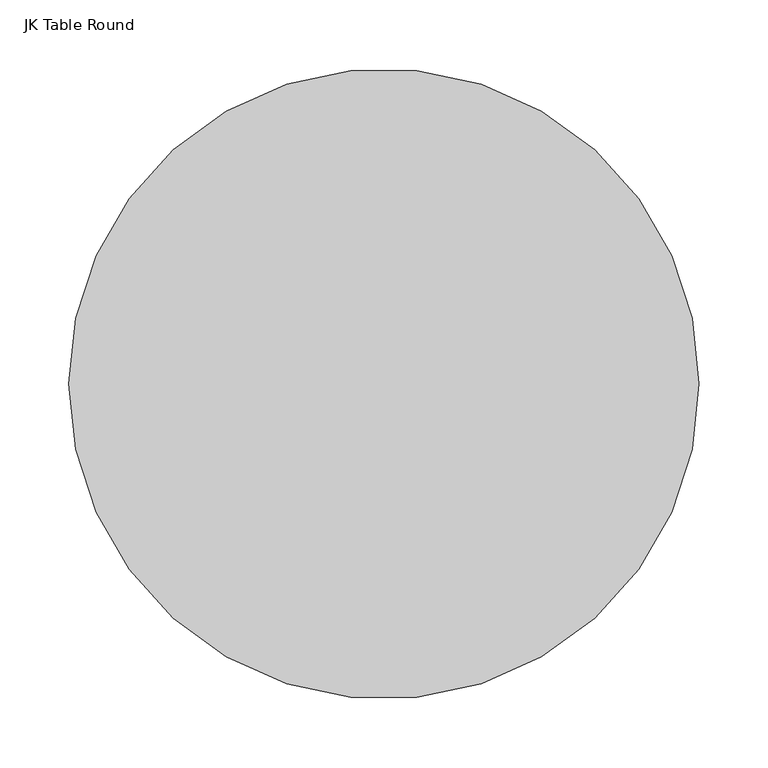
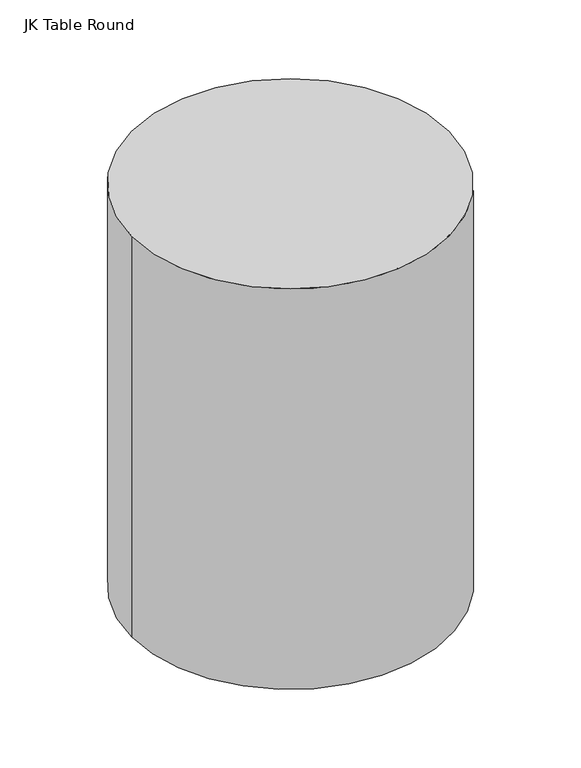
"""IFC4 building model written with IfcOpenShell, lengths in millimetres: furniture geometry, JK Table Round : Counsel End Table."""

import ifcopenshell
import ifcopenshell.guid

model = None  # the IFC model being written
_history = None  # IfcOwnerHistory: only IFC2X3 demands one
_inside = {}  # id of a spatial element -> (the spatial element, [elements in it])
_under = {}  # id of a project, library or spatial element -> (it, [spatial elements below it])
_declared = {}  # id of a project -> (the project, [libraries it declares])
_typed = {}  # id of a type object -> (the type object, [elements of that type])
_made_of = {}  # id of a material, layer set ... -> (it, [elements and type objects made of it])


def new_model(schema):
    """Start an empty IFC model of exactly this schema.

    Asked for "IFC4X3", IfcOpenShell would pick the latest addendum, in which some entities
    have other attributes; the version numbers below select the first issue.
    IFC2X3 requires an IfcOwnerHistory on every rooted entity: one is made here for all.
    """
    global model, _history
    if schema == "IFC4X3":
        model = ifcopenshell.file(schema_version=(4, 3, 0, 0))
    else:
        model = ifcopenshell.file(schema=schema)
    _inside.clear()
    _under.clear()
    _declared.clear()
    _typed.clear()
    _made_of.clear()
    _history = None
    if model.schema == "IFC2X3":
        org = make("IfcOrganization", Name="unknown")
        user = make(
            "IfcPersonAndOrganization",
            ThePerson=make("IfcPerson", FamilyName="unknown"),
            TheOrganization=org,
        )
        app = make(
            "IfcApplication",
            ApplicationDeveloper=org,
            Version="unknown",
            ApplicationFullName="unknown",
            ApplicationIdentifier="unknown",
        )
        _history = make(
            "IfcOwnerHistory",
            OwningUser=user,
            OwningApplication=app,
            ChangeAction="ADDED",
            CreationDate=0,
        )
    return model


def make(cls, **values):
    """One entity of the class cls with the attributes given. An attribute that is None is left unset."""
    return model.create_entity(
        cls, **{name: value for name, value in values.items() if value is not None}
    )


def rooted(cls, **values):
    """An entity with a GlobalId (a new one), such as an element, a storey or a relation."""
    return make(cls, GlobalId=ifcopenshell.guid.new(), OwnerHistory=_history, **values)


def si_unit(unit_type, name, prefix=None):
    """IfcSIUnit, for example si_unit("LENGTHUNIT", "METRE", prefix="MILLI")."""
    return make("IfcSIUnit", UnitType=unit_type, Prefix=prefix, Name=name)


def assignment(units):
    """IfcUnitAssignment: the units of a project."""
    return None if units is None else make("IfcUnitAssignment", Units=units)


def point(xyz):
    """IfcCartesianPoint."""
    return None if xyz is None else make("IfcCartesianPoint", Coordinates=xyz)


def direction(xyz):
    """IfcDirection."""
    return None if xyz is None else make("IfcDirection", DirectionRatios=xyz)


def frame(location, z_axis=None, x_axis=None):
    """IfcAxis2Placement3D, a coordinate frame: its origin and axes. An axis left out is left unset."""
    return make(
        "IfcAxis2Placement3D",
        Location=point(location),
        Axis=direction(z_axis),
        RefDirection=direction(x_axis),
    )


def frame_2d(location, x_axis=None):
    """IfcAxis2Placement2D, a coordinate frame in the plane: its origin and x axis."""
    return make(
        "IfcAxis2Placement2D", Location=point(location), RefDirection=direction(x_axis)
    )


def origin():
    """The frame at (0, 0, 0) with its axes left unset."""
    return frame((0.0, 0.0, 0.0))


def origin_with_axes():
    """The frame at (0, 0, 0) with the z axis (0, 0, 1) and the x axis (1, 0, 0) written out."""
    return frame((0.0, 0.0, 0.0), z_axis=(0.0, 0.0, 1.0), x_axis=(1.0, 0.0, 0.0))


def place(relative_to, where):
    """IfcLocalPlacement: puts the frame where relative to a parent placement (None: the world)."""
    return make(
        "IfcLocalPlacement", PlacementRelTo=relative_to, RelativePlacement=where
    )


def context(
    kind, dimensions, precision=None, world=None, true_north=None, identifier=None
):
    """IfcGeometricRepresentationContext, for example the 3D "Model" context."""
    return make(
        "IfcGeometricRepresentationContext",
        ContextIdentifier=identifier,
        ContextType=kind,
        CoordinateSpaceDimension=dimensions,
        Precision=precision,
        WorldCoordinateSystem=world,
        TrueNorth=true_north,
    )


def project(units=None, contexts=None):
    """IfcProject with its units and contexts."""
    return rooted(
        "IfcProject",
        Name="project",
        RepresentationContexts=contexts,
        UnitsInContext=assignment(units),
    )


def spatial(cls, under=None, at=None, **own):
    """A site, building, storey or space (cls), placed at a placement, below another one or the project."""
    s = rooted(cls, ObjectPlacement=at, **own)
    if under is not None:
        _under.setdefault(under.id(), (under, []))[1].append(s)
    return s


def circle_curve(where, radius):
    """IfcCircle in the frame where."""
    return make("IfcCircle", Position=where, Radius=radius)


def trimmed(basis, trim1, trim2, sense, master):
    """IfcTrimmedCurve: the piece of a basis curve between two trims."""
    return make(
        "IfcTrimmedCurve",
        BasisCurve=basis,
        Trim1=trim1,
        Trim2=trim2,
        SenseAgreement=sense,
        MasterRepresentation=master,
    )


def segment(curve, same_sense, transition):
    """IfcCompositeCurveSegment."""
    return make(
        "IfcCompositeCurveSegment",
        Transition=transition,
        SameSense=same_sense,
        ParentCurve=curve,
    )


def composite_curve(segments, self_intersect=None):
    """IfcCompositeCurve: segments joined end to end."""
    return make("IfcCompositeCurve", Segments=segments, SelfIntersect=self_intersect)


def outline(outer, holes=None, kind="AREA"):
    """IfcArbitraryClosedProfileDef: a profile drawn as a closed curve; with holes, ...WithVoids."""
    if holes is None:
        return make("IfcArbitraryClosedProfileDef", ProfileType=kind, OuterCurve=outer)
    return make(
        "IfcArbitraryProfileDefWithVoids",
        ProfileType=kind,
        OuterCurve=outer,
        InnerCurves=holes,
    )


def extrude(swept, where, along, depth):
    """IfcExtrudedAreaSolid: the profile swept, set in the frame where, extruded along a direction by depth."""
    return make(
        "IfcExtrudedAreaSolid",
        SweptArea=swept,
        Position=where,
        ExtrudedDirection=direction(along),
        Depth=depth,
    )


def shape(context_of_items, identifier, shape_type, items):
    """IfcShapeRepresentation: the items that make up one representation, for example the "Body"."""
    return make(
        "IfcShapeRepresentation",
        ContextOfItems=context_of_items,
        RepresentationIdentifier=identifier,
        RepresentationType=shape_type,
        Items=items,
    )


def source(mapping_origin, context_of_items, identifier, shape_type, items):
    """IfcRepresentationMap: a shape defined once, which mapped items show again and again."""
    return make(
        "IfcRepresentationMap",
        MappingOrigin=mapping_origin,
        MappedRepresentation=shape(context_of_items, identifier, shape_type, items),
    )


def transform(
    local_origin,
    x_axis=None,
    y_axis=None,
    z_axis=None,
    scale=None,
    scale2=None,
    scale3=None,
    uniform=True,
):
    """IfcCartesianTransformationOperator3D, or its non-uniform kind. x_axis, y_axis, z_axis: its Axis1, 2, 3."""
    if uniform:
        return make(
            "IfcCartesianTransformationOperator3D",
            Axis1=direction(x_axis),
            Axis2=direction(y_axis),
            LocalOrigin=point(local_origin),
            Scale=scale,
            Axis3=direction(z_axis),
        )
    return make(
        "IfcCartesianTransformationOperator3DnonUniform",
        Axis1=direction(x_axis),
        Axis2=direction(y_axis),
        LocalOrigin=point(local_origin),
        Scale=scale,
        Axis3=direction(z_axis),
        Scale2=scale2,
        Scale3=scale3,
    )


def mapped(mapping_source, mapping_target):
    """IfcMappedItem: shows the shape of a source again, moved by a transform."""
    return make(
        "IfcMappedItem", MappingSource=mapping_source, MappingTarget=mapping_target
    )


def made_of(thing, what):
    """Note that an element or type object is made of a material, layer set ...; save() writes the relation."""
    if what is not None:
        _made_of.setdefault(what.id(), (what, []))[1].append(thing)
    return thing


def element(
    cls,
    number,
    at=None,
    inside=None,
    cuts=None,
    type_object=None,
    material=None,
    context=None,
    identifier="Body",
    shape_type=None,
    held_by="IfcProductDefinitionShape",
    body=None,
    shapes=None,
    **own,
):
    """One element of the class cls, such as IfcWall. Its Tag is "e" and its number.

    at: its placement. inside: the storey or other place that contains it. cuts: it is an
    opening in that element (IfcRelVoidsElement). A single representation is given by context,
    identifier, shape_type and body (its items); several are given by shapes. held_by: the class
    of the entity that holds the representations. save() writes the other relations.
    """
    e = rooted(cls, Tag="e%d" % number, ObjectPlacement=at, **own)
    if body is not None:
        shapes = [shape(context, identifier, shape_type, body)]
    if shapes is not None:
        e.Representation = make(held_by, Representations=shapes)
    if inside is not None:
        _inside.setdefault(inside.id(), (inside, []))[1].append(e)
    if cuts is not None:
        rooted(
            "IfcRelVoidsElement", RelatingBuildingElement=cuts, RelatedOpeningElement=e
        )
    if type_object is not None:
        _typed.setdefault(type_object.id(), (type_object, []))[1].append(e)
    return made_of(e, material)


def aggregate(whole, parts):
    """IfcRelAggregates: a whole, such as a stair, and the parts it consists of."""
    return rooted("IfcRelAggregates", RelatingObject=whole, RelatedObjects=parts)


def save(model, path):
    """Write the relations noted so far, then the file.

    IfcRelAggregates (storeys below a building ...), IfcRelContainedInSpatialStructure (elements
    in a storey), IfcRelDefinesByType, IfcRelAssociatesMaterial and IfcRelDeclares: one each for
    every whole, place, type object, material and project.
    """
    for whole, parts in _under.values():
        aggregate(whole, parts)
    for where, things in _inside.values():
        rooted(
            "IfcRelContainedInSpatialStructure",
            RelatedElements=things,
            RelatingStructure=where,
        )
    for kind, things in _typed.values():
        rooted("IfcRelDefinesByType", RelatedObjects=things, RelatingType=kind)
    for what, things in _made_of.values():
        rooted("IfcRelAssociatesMaterial", RelatedObjects=things, RelatingMaterial=what)
    for by, libraries in _declared.values():
        rooted("IfcRelDeclares", RelatingContext=by, RelatedDefinitions=libraries)
    model.write(path)


def jk_table_round_4d053911(model_context):
    return source(origin(), model_context, "Body", "SweptSolid", [
        extrude(outline(composite_curve([segment(trimmed(circle_curve(frame_2d((-61.9426335, -33.5455296)), 228.6), [point((-290.5426335, -33.5455296))], [point((166.6573665, -33.5455296))], False, "CARTESIAN"), True, "CONTINUOUS"), segment(trimmed(circle_curve(frame_2d((-61.9426335, -33.5455296)), 228.6), [point((166.6573665, -33.5455296))], [point((-290.5426335, -33.5455296))], False, "CARTESIAN"), True, "CONTINUOUS")], self_intersect=False)), origin_with_axes(), (0.0, 0.0, 1.0), 609.6),
    ])


if __name__ == "__main__":
    model = new_model("IFC4")
    model_context = context("Model", 3, world=origin())
    ifc_project = project(units=[si_unit("LENGTHUNIT", "METRE", prefix="MILLI")], contexts=[model_context])
    site = spatial("IfcSite", under=ifc_project)
    building = spatial("IfcBuilding", under=site)
    placement = place(None, origin())
    jk_table_round_shape = jk_table_round_4d053911(model_context)
    element("IfcFurniture", 1, ObjectType="JK Table Round : Counsel End Table", at=placement, inside=building, context=model_context, shape_type="MappedRepresentation", body=[
        mapped(jk_table_round_shape, transform((0.0, 0.0, 0.0), x_axis=(1.0, 0.0, 0.0), y_axis=(0.0, 1.0, 0.0), z_axis=(0.0, 0.0, 1.0))),
    ])
    save(model, "model.ifc")

# Revit data of these elements
# Type "JK Table Round : Counsel End Table"
#   Width = 1' - 6"
#   Height = 2' - 0"
#   Status [instance default] = none
#   Default Elevation = 0
